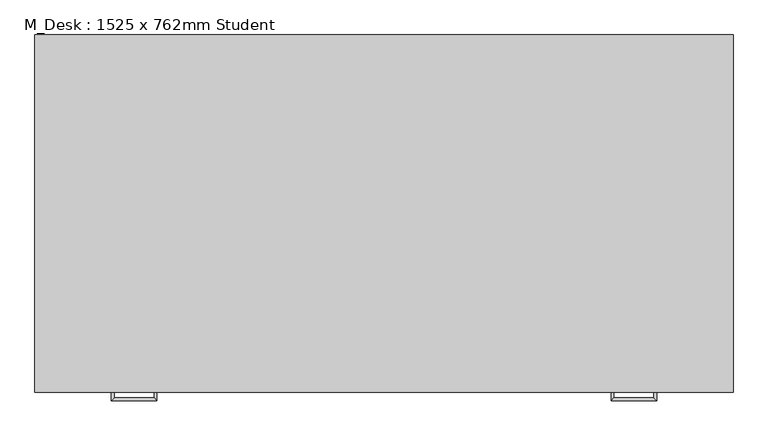
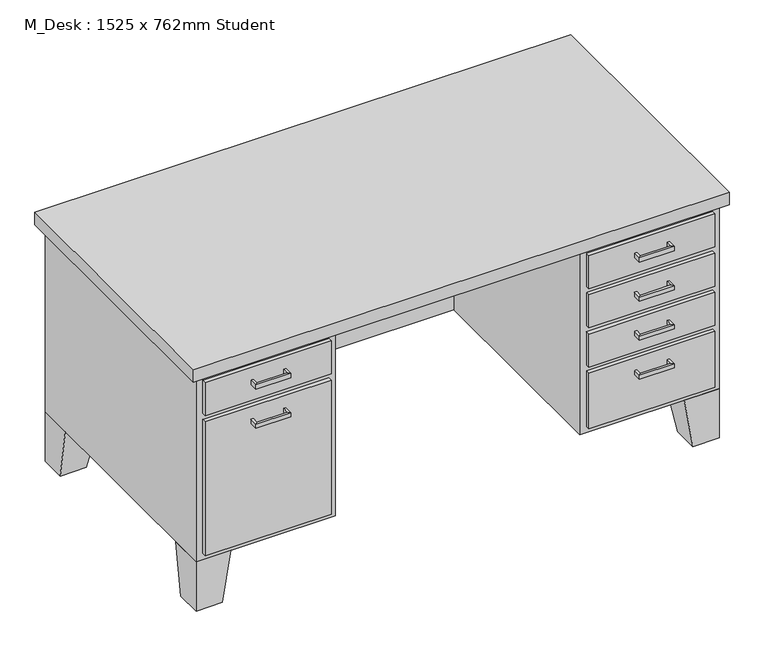
"""IFC4 building model written with IfcOpenShell, lengths in millimetres: furniture geometry, M_Desk : 1525 x 762mm Student."""

from ifc_helpers import new_model, si_unit, frame, origin, place, context, project, spatial, polyline, outline, extrude, faceted_brep, source, transform, mapped, element, save


def m_desk_1525_x_762mm_student_34485ced(model_context):
    return source(origin(), model_context, "Body", "SolidModel", [
        extrude(outline(polyline([(1118.1, 0.0), (1118.1, 635.0), (405.9, 635.0), (405.9, 0.0), (-0.5, 0.0), (-0.5, 762.0), (1524.5, 762.0), (1524.5, 0.0), (1118.1, 0.0)])), frame((0.0, 0.0, 152.0), z_axis=(0.0, 0.0, 1.0), x_axis=(1.0, 0.0, 0.0)), (0.0, 0.0, 1.0), 571.9),
        extrude(outline(polyline([(-19.55, -19.05), (-19.55, 781.05), (1543.55, 781.05), (1543.55, -19.05), (-19.55, -19.05)])), frame((0.0, 0.0, 723.9), z_axis=(0.0, 0.0, 1.0), x_axis=(1.0, 0.0, 0.0)), (0.0, 0.0, 1.0), 38.1),
        faceted_brep([(1422.9, 0.0, 152.0), (1524.5, 0.0, 152.0), (1524.5, 101.6, 152.0), (1422.9, 101.6, 152.0), (1448.3, 0.0, 0.0), (1448.3, 76.2, 0.0), (1524.5, 76.2, 0.0), (1524.5, 0.0, 0.0)], [[[0, 1, 2, 3]], [[4, 5, 6, 7]], [[4, 7, 1, 0]], [[7, 6, 2, 1]], [[6, 5, 3, 2]], [[5, 4, 0, 3]]]),
        faceted_brep([(1422.9, 762.0, 152.0), (1422.9, 660.4, 152.0), (1524.5, 660.4, 152.0), (1524.5, 762.0, 152.0), (1448.3, 762.0, 0.0), (1524.5, 762.0, 0.0), (1524.5, 685.8, 0.0), (1448.3, 685.8, 0.0)], [[[0, 1, 2, 3]], [[4, 5, 6, 7]], [[4, 7, 1, 0]], [[7, 6, 2, 1]], [[6, 5, 3, 2]], [[5, 4, 0, 3]]]),
        faceted_brep([(101.1, 762.0, 152.0), (-0.5, 762.0, 152.0), (-0.5, 660.4, 152.0), (101.1, 660.4, 152.0), (75.7, 762.0, 0.0), (75.7, 685.8, 0.0), (-0.5, 685.8, 0.0), (-0.5, 762.0, 0.0)], [[[0, 1, 2, 3]], [[4, 5, 6, 7]], [[4, 7, 1, 0]], [[7, 6, 2, 1]], [[6, 5, 3, 2]], [[5, 4, 0, 3]]]),
        faceted_brep([(101.1, 0.0, 152.0), (101.1, 101.6, 152.0), (-0.5, 101.6, 152.0), (-0.5, 0.0, 152.0), (75.7, 0.0, 0.0), (-0.5, 0.0, 0.0), (-0.5, 76.2, 0.0), (75.7, 76.2, 0.0)], [[[0, 1, 2, 3]], [[4, 5, 6, 7]], [[4, 7, 1, 0]], [[7, 6, 2, 1]], [[6, 5, 3, 2]], [[5, 4, 0, 3]]]),
        extrude(outline(polyline([(1137.15, 0.0), (1505.45, 0.0), (1505.45, -12.7), (1137.15, -12.7), (1137.15, 0.0)])), frame((0.0, 0.0, 602.85), z_axis=(0.0, 0.0, 1.0), x_axis=(1.0, 0.0, 0.0)), (0.0, 0.0, 1.0), 102.0),
        extrude(outline(polyline([(1137.15, 0.0), (1505.45, 0.0), (1505.45, -12.7), (1137.15, -12.7), (1137.15, 0.0)])), frame((0.0, 0.0, 171.05), z_axis=(0.0, 0.0, 1.0), x_axis=(1.0, 0.0, 0.0)), (0.0, 0.0, 1.0), 171.45),
        extrude(outline(polyline([(1137.15, 0.0), (1505.45, 0.0), (1505.45, -12.7), (1137.15, -12.7), (1137.15, 0.0)])), frame((0.0, 0.0, 482.2), z_axis=(0.0, 0.0, 1.0), x_axis=(1.0, 0.0, 0.0)), (0.0, 0.0, 1.0), 101.6),
        extrude(outline(polyline([(1137.15, 0.0), (1505.45, 0.0), (1505.45, -12.7), (1137.15, -12.7), (1137.15, 0.0)])), frame((0.0, 0.0, 361.55), z_axis=(0.0, 0.0, 1.0), x_axis=(1.0, 0.0, 0.0)), (0.0, 0.0, 1.0), 101.6),
        extrude(outline(polyline([(18.55, 0.0), (386.85, 0.0), (386.85, -12.7), (18.55, -12.7), (18.55, 0.0)])), frame((0.0, 0.0, 603.25), z_axis=(0.0, 0.0, 1.0), x_axis=(1.0, 0.0, 0.0)), (0.0, 0.0, 1.0), 101.6),
        extrude(outline(polyline([(18.55, 0.0), (386.85, 0.0), (386.85, -12.7), (18.55, -12.7), (18.55, 0.0)])), frame((0.0, 0.0, 171.05), z_axis=(0.0, 0.0, 1.0), x_axis=(1.0, 0.0, 0.0)), (0.0, 0.0, 1.0), 413.15),
        faceted_brep([(1365.75, -12.7, 304.8), (1372.1, -12.7, 304.8), (1372.1, -12.7, 292.1), (1365.75, -12.7, 292.1), (1365.75, -31.75, 304.8), (1372.1, -38.1, 304.8), (1372.1, -38.1, 292.1), (1365.75, -31.75, 292.1), (1276.85, -31.75, 304.8), (1270.5, -38.1, 304.8), (1270.5, -38.1, 292.1), (1276.85, -31.75, 292.1), (1276.85, -12.7, 304.8), (1276.85, -12.7, 292.1), (1270.5, -12.7, 292.1), (1270.5, -12.7, 304.8)], [[[0, 1, 2, 3]], [[1, 0, 4, 5]], [[2, 1, 5, 6]], [[3, 2, 6, 7]], [[0, 3, 7, 4]], [[5, 4, 8, 9]], [[6, 5, 9, 10]], [[7, 6, 10, 11]], [[4, 7, 11, 8]], [[12, 13, 14, 15]], [[9, 8, 12, 15]], [[10, 9, 15, 14]], [[11, 10, 14, 13]], [[8, 11, 13, 12]]]),
        faceted_brep([(1365.75, -12.7, 425.45), (1372.1, -12.7, 425.45), (1372.1, -12.7, 412.75), (1365.75, -12.7, 412.75), (1365.75, -31.75, 425.45), (1372.1, -38.1, 425.45), (1372.1, -38.1, 412.75), (1365.75, -31.75, 412.75), (1276.85, -31.75, 425.45), (1270.5, -38.1, 425.45), (1270.5, -38.1, 412.75), (1276.85, -31.75, 412.75), (1276.85, -12.7, 425.45), (1276.85, -12.7, 412.75), (1270.5, -12.7, 412.75), (1270.5, -12.7, 425.45)], [[[0, 1, 2, 3]], [[1, 0, 4, 5]], [[2, 1, 5, 6]], [[3, 2, 6, 7]], [[0, 3, 7, 4]], [[5, 4, 8, 9]], [[6, 5, 9, 10]], [[7, 6, 10, 11]], [[4, 7, 11, 8]], [[12, 13, 14, 15]], [[9, 8, 12, 15]], [[10, 9, 15, 14]], [[11, 10, 14, 13]], [[8, 11, 13, 12]]]),
        faceted_brep([(1365.75, -12.7, 546.1), (1372.1, -12.7, 546.1), (1372.1, -12.7, 533.4), (1365.75, -12.7, 533.4), (1365.75, -31.75, 546.1), (1372.1, -38.1, 546.1), (1372.1, -38.1, 533.4), (1365.75, -31.75, 533.4), (1276.85, -31.75, 546.1), (1270.5, -38.1, 546.1), (1270.5, -38.1, 533.4), (1276.85, -31.75, 533.4), (1276.85, -12.7, 546.1), (1276.85, -12.7, 533.4), (1270.5, -12.7, 533.4), (1270.5, -12.7, 546.1)], [[[0, 1, 2, 3]], [[1, 0, 4, 5]], [[2, 1, 5, 6]], [[3, 2, 6, 7]], [[0, 3, 7, 4]], [[5, 4, 8, 9]], [[6, 5, 9, 10]], [[7, 6, 10, 11]], [[4, 7, 11, 8]], [[12, 13, 14, 15]], [[9, 8, 12, 15]], [[10, 9, 15, 14]], [[11, 10, 14, 13]], [[8, 11, 13, 12]]]),
        faceted_brep([(1365.75, -12.7, 666.75), (1372.1, -12.7, 666.75), (1372.1, -12.7, 654.05), (1365.75, -12.7, 654.05), (1365.75, -31.75, 666.75), (1372.1, -38.1, 666.75), (1372.1, -38.1, 654.05), (1365.75, -31.75, 654.05), (1276.85, -31.75, 666.75), (1270.5, -38.1, 666.75), (1270.5, -38.1, 654.05), (1276.85, -31.75, 654.05), (1276.85, -12.7, 666.75), (1276.85, -12.7, 654.05), (1270.5, -12.7, 654.05), (1270.5, -12.7, 666.75)], [[[0, 1, 2, 3]], [[1, 0, 4, 5]], [[2, 1, 5, 6]], [[3, 2, 6, 7]], [[0, 3, 7, 4]], [[5, 4, 8, 9]], [[6, 5, 9, 10]], [[7, 6, 10, 11]], [[4, 7, 11, 8]], [[12, 13, 14, 15]], [[9, 8, 12, 15]], [[10, 9, 15, 14]], [[11, 10, 14, 13]], [[8, 11, 13, 12]]]),
        faceted_brep([(158.25, -12.7, 546.1), (158.25, -12.7, 533.4), (151.9, -12.7, 533.4), (151.9, -12.7, 546.1), (158.25, -31.75, 546.1), (158.25, -31.75, 533.4), (151.9, -38.1, 533.4), (151.9, -38.1, 546.1), (247.15, -31.75, 546.1), (247.15, -31.75, 533.4), (253.5, -38.1, 533.4), (253.5, -38.1, 546.1), (247.15, -12.7, 546.1), (253.5, -12.7, 546.1), (253.5, -12.7, 533.4), (247.15, -12.7, 533.4)], [[[0, 1, 2, 3]], [[1, 0, 4, 5]], [[2, 1, 5, 6]], [[3, 2, 6, 7]], [[0, 3, 7, 4]], [[5, 4, 8, 9]], [[6, 5, 9, 10]], [[7, 6, 10, 11]], [[4, 7, 11, 8]], [[12, 13, 14, 15]], [[9, 8, 12, 15]], [[10, 9, 15, 14]], [[11, 10, 14, 13]], [[8, 11, 13, 12]]]),
        faceted_brep([(158.25, -12.7, 666.75), (158.25, -12.7, 654.05), (151.9, -12.7, 654.05), (151.9, -12.7, 666.75), (158.25, -31.75, 666.75), (158.25, -31.75, 654.05), (151.9, -38.1, 654.05), (151.9, -38.1, 666.75), (247.15, -31.75, 666.75), (247.15, -31.75, 654.05), (253.5, -38.1, 654.05), (253.5, -38.1, 666.75), (247.15, -12.7, 666.75), (253.5, -12.7, 666.75), (253.5, -12.7, 654.05), (247.15, -12.7, 654.05)], [[[0, 1, 2, 3]], [[1, 0, 4, 5]], [[2, 1, 5, 6]], [[3, 2, 6, 7]], [[0, 3, 7, 4]], [[5, 4, 8, 9]], [[6, 5, 9, 10]], [[7, 6, 10, 11]], [[4, 7, 11, 8]], [[12, 13, 14, 15]], [[9, 8, 12, 15]], [[10, 9, 15, 14]], [[11, 10, 14, 13]], [[8, 11, 13, 12]]]),
    ])


if __name__ == "__main__":
    model = new_model("IFC4")
    model_context = context("Model", 3, world=origin())
    ifc_project = project(units=[si_unit("LENGTHUNIT", "METRE", prefix="MILLI")], contexts=[model_context])
    site = spatial("IfcSite", under=ifc_project)
    building = spatial("IfcBuilding", under=site)
    placement = place(None, origin())
    m_desk_1525_x_762mm_student_shape = m_desk_1525_x_762mm_student_34485ced(model_context)
    element("IfcFurniture", 1, ObjectType="M_Desk : 1525 x 762mm Student", at=placement, inside=building, context=model_context, shape_type="MappedRepresentation", body=[
        mapped(m_desk_1525_x_762mm_student_shape, transform((0.0, 0.0, 0.0), x_axis=(1.0, 0.0, 0.0), y_axis=(0.0, 1.0, 0.0), z_axis=(0.0, 0.0, 1.0))),
    ])
    save(model, "model.ifc")

# Revit data of these elements
# Type "M_Desk : 1525 x 762mm Student"
#   Depth = 762 mm
#   Height = 762 mm
#   Leg Height = 152 mm
#   Width = 1525 mm
#   Body Material = Laminate, Ivory, Matte
#   Handle/Leg Material = Steel, Chrome Plated
#   Top Material = Cherry
#   Default Elevation = 0
# Element 1 (IfcFurniture, "M_Desk : 1525 x 762mm Student")
#   Materials on its faces: "Steel, Chrome Plated", "Laminate, Ivory, Matte", "Cherry"
# Materials
#   "Laminate, Ivory, Matte": class "Plastic", colour RGB 244 244 244, transparency 0, Description = "Plastic Laminate - Ivory, Matte", Cost = 0
#   "Steel, Chrome Plated": class "Metal", colour RGB 17 17 17, transparency 0, Description = "Chromiuim plated steel", Cost = 0
#   "Cherry": class "Wood", colour RGB 158 77 40, transparency 0, Description = "Prunus Serotina", Cost = 0
